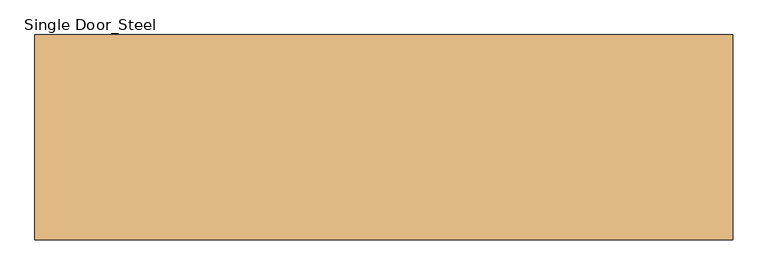
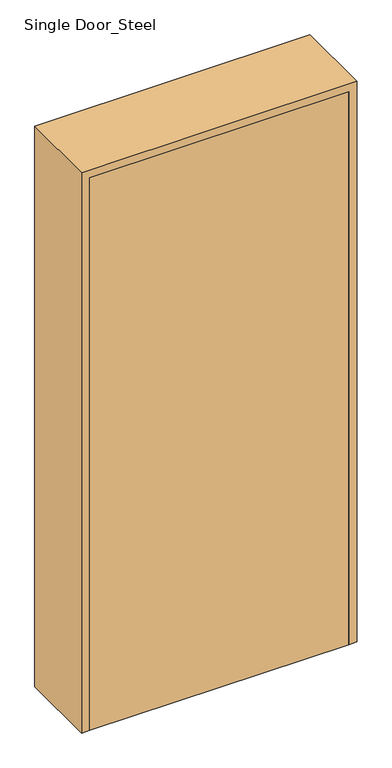
"""IFC4 building model written with IfcOpenShell, lengths in millimetres: door geometry, Single Door_Steel : H_DR_AMB_Single Door_Steel_W1000xH2150."""

from ifc_helpers import new_model, si_unit, origin, origin_with_axes, place, context, project, spatial, polyline, outline, extrude, faceted_brep, source, transform, mapped, element, save


def single_door_steel_221a647d(model_context):
    return source(origin(), model_context, "Body", "SolidModel", [
        extrude(outline(polyline([(470.0, -147.0), (-470.0, -147.0), (-470.0, -112.0), (470.0, -112.0), (470.0, -147.0)])), origin_with_axes(), (0.0, 0.0, 1.0), 2120.0),
        faceted_brep([(470.0, -147.0, 0.0), (470.0, -112.0, 0.0), (450.0, -112.0, 0.0), (450.0, 112.0, 0.0), (470.0, 112.0, 0.0), (470.0, 147.0, 0.0), (500.0, 147.0, 0.0), (500.0, -147.0, 0.0), (500.0, -147.0, 2150.0), (-500.0, -147.0, 2150.0), (-500.0, -147.0, 0.0), (-470.0, -147.0, 0.0), (-470.0, -147.0, 2120.0), (470.0, -147.0, 2120.0), (500.0, 147.0, 2150.0), (470.0, 147.0, 2120.0), (-470.0, 147.0, 2120.0), (-470.0, 147.0, 0.0), (-500.0, 147.0, 0.0), (-500.0, 147.0, 2150.0), (470.0, 112.0, 2120.0), (450.0, 112.0, 2100.0), (-450.0, 112.0, 2100.0), (-450.0, 112.0, 0.0), (-470.0, 112.0, 0.0), (-470.0, 112.0, 2120.0), (450.0, -112.0, 2100.0), (470.0, -112.0, 2120.0), (-470.0, -112.0, 2120.0), (-470.0, -112.0, 0.0), (-450.0, -112.0, 0.0), (-450.0, -112.0, 2100.0)], [[[0, 1, 2, 3, 4, 5, 6, 7]], [[7, 8, 9, 10, 11, 12, 13, 0]], [[6, 14, 8, 7]], [[5, 15, 16, 17, 18, 19, 14, 6]], [[4, 20, 15, 5]], [[3, 21, 22, 23, 24, 25, 20, 4]], [[2, 26, 21, 3]], [[1, 27, 28, 29, 30, 31, 26, 2]], [[0, 13, 27, 1]], [[12, 11, 29, 28]], [[11, 10, 18, 17, 24, 23, 30, 29]], [[19, 18, 10, 9]], [[25, 24, 17, 16]], [[31, 30, 23, 22]], [[14, 19, 9, 8]], [[20, 25, 16, 15]], [[26, 31, 22, 21]], [[13, 12, 28, 27]]]),
    ])


if __name__ == "__main__":
    model = new_model("IFC4")
    model_context = context("Model", 3, world=origin())
    ifc_project = project(units=[si_unit("LENGTHUNIT", "METRE", prefix="MILLI")], contexts=[model_context])
    site = spatial("IfcSite", under=ifc_project)
    building = spatial("IfcBuilding", under=site)
    placement = place(None, origin())
    single_door_steel_shape = single_door_steel_221a647d(model_context)
    element("IfcDoor", 1, ObjectType="Single Door_Steel : H_DR_AMB_Single Door_Steel_W1000xH2150", at=placement, inside=building, context=model_context, shape_type="MappedRepresentation", body=[
        mapped(single_door_steel_shape, transform((0.0, 0.0, 0.0), x_axis=(1.0, 0.0, 0.0), y_axis=(0.0, 1.0, 0.0), z_axis=(0.0, 0.0, 1.0))),
    ])
    save(model, "model.ifc")

# Revit data of these elements
# Type "Single Door_Steel : H_DR_AMB_Single Door_Steel_W1000xH2150"
#   Type Mark = "364"
#   Analytic Construction = "<None>"
#   프레임 투영 외부. = 25.000 mm
#   프레임 투영 내부. = 25.000 mm
#   프레임 폭 = 75.000 mm
#   Height = 2150.000 mm
#   Width = 1000.000 mm
#   Define Thermal Properties by = 1
#   문 패널 = none
#   문 프레임 = none
#   Function = (empty or 0)
#   Wall Closure = (empty or 0)
